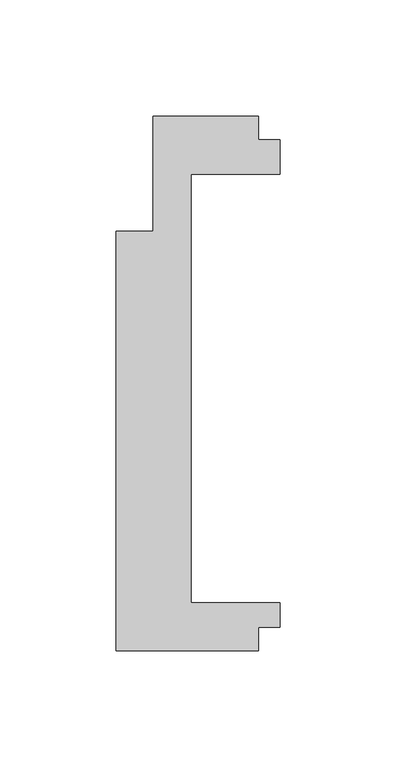
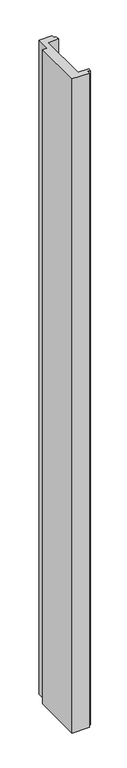
"""IFC4 building model written with IfcOpenShell, lengths in millimetres: proxy geometry, Generic Models 7:Generic Models 1:337419:Generic Models 1:337419 : Generic Models 7:Generic Models 1:337419:52 : Generic Models 7:Generic Models 1:337419:Generic Models 1:337419 : Generic Models 7:Generic Models 1:337419:301336."""

from ifc_helpers import new_model, si_unit, origin, origin_with_axes, place, context, project, spatial, polyline, outline, extrude, source, transform, mapped, element, save


def generic_models_426fa44d(model_context):
    return source(origin(), model_context, "Body", "SweptSolid", [
        extrude(outline(polyline([(593789.2835992, -536560.0694608), (593789.2835992, -536569.9913358), (593798.4117242, -536569.9913358), (593798.4117242, -536584.8076082), (593760.3117242, -536584.8076082), (593760.3117242, -536768.9576082), (593798.4117242, -536768.9576082), (593798.4117242, -536779.5413358), (593789.2835992, -536779.5413358), (593789.2835992, -536789.4632108), (593728.1648492, -536789.4632108), (593728.1648492, -536609.2819608), (593744.0398492, -536609.2819608), (593744.0398492, -536560.0694608), (593789.2835992, -536560.0694608)])), origin_with_axes(), (0.0, 0.0, 1.0), 2438.4),
    ])


if __name__ == "__main__":
    model = new_model("IFC4")
    model_context = context("Model", 3, world=origin())
    ifc_project = project(units=[si_unit("LENGTHUNIT", "METRE", prefix="MILLI")], contexts=[model_context])
    site = spatial("IfcSite", under=ifc_project)
    building = spatial("IfcBuilding", under=site)
    placement = place(None, origin())
    generic_models_shape = generic_models_426fa44d(model_context)
    element("IfcBuildingElementProxy", 1, Name="Generic Models 7:Generic Models 1:337419:Generic Models 1:337419 : Generic Models 7:Generic Models 1:337419:52 : Generic Models 7:Generic Models 1:337419:Generic Models 1:337419 : Generic Models 7:Generic Models 1:337419:301336", ObjectType="Generic Models 7:Generic Models 1:337419:Generic Models 1:337419 : Generic Models 7:Generic Models 1:337419:52 : Generic Models 7:Generic Models 1:337419:Generic Models 1:337419 : Generic Models 7:Generic Models 1:337419:301336", at=placement, inside=building, context=model_context, shape_type="MappedRepresentation", body=[
        mapped(generic_models_shape, transform((0.0, 0.0, 0.0), x_axis=(1.0, 0.0, 0.0), y_axis=(0.0, 1.0, 0.0), z_axis=(0.0, 0.0, 1.0))),
    ])
    save(model, "model.ifc")

# Revit data of these elements
# Type "Generic Models 7:Generic Models 1:337419:Generic Models 1:337419 : Generic Models 7:Generic Models 1:337419:52 : Generic Models 7:Generic Models 1:337419:Generic Models 1:337419 : Generic Models 7:Generic Models 1:337419:301336"
#   NameOverride = "Generic Models 7:Generic Models 1:337419:Generic Models 1:337419 : Generic Models 7:Generic Models 1:337419:301336"
#   ObjectTypeOverride = "Generic Models 1:337419 : Generic Models 7:Generic Models 1:337419"
#   Reference = "Generic Models 1"
#   Tag = "301336"
# Element 1 (IfcBuildingElementProxy, "Generic Models 7:Generic Models 1:337419:Generic Models 1:337419 : Generic Models 7:Generic Models 1:337419:52 : Generic Models 7:Generic Models 1:337419:Generic Models 1:337419 : Generic Models 7:Generic Models 1:337419:301336")
#   Materials on its faces: "LOW VOLUMN EXPANDABLE FOAM INSULATION (CLASS A FLAME SPREAD)"
# Materials
#   "LOW VOLUMN EXPANDABLE FOAM INSULATION (CLASS A FLAME SPREAD)": class "Unassigned", colour RGB 213 216 95, transparency 0, Cost = 0
